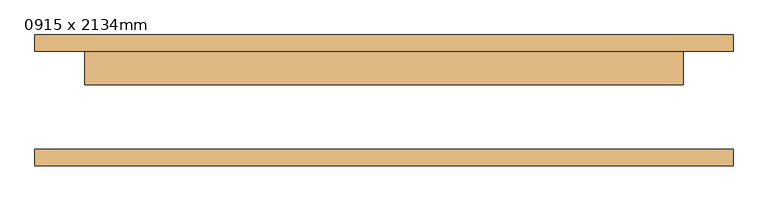
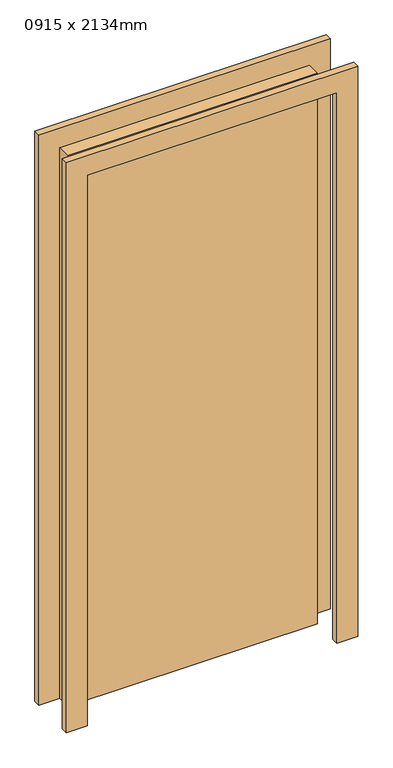
"""IFC4 building model written with IfcOpenShell, lengths in millimetres: door geometry, M_Folha única : 0915 x 2134mm."""

from ifc_helpers import new_model, si_unit, frame, origin, origin_with_axes, place, context, project, spatial, polyline, outline, extrude, source, transform, mapped, element, save


def door_0915_x_2134mm_138fd904(model_context):
    return source(origin(), model_context, "Body", "SweptSolid", [
        extrude(outline(polyline([(2210.0, -533.5), (0.0, -533.5), (0.0, -457.5), (2134.0, -457.5), (2134.0, 457.5), (0.0, 457.5), (0.0, 533.5), (2210.0, 533.5), (2210.0, -533.5)])), frame((0.0, 75.0, 0.0), z_axis=(0.0, 1.0, 0.0), x_axis=(0.0, 0.0, 1.0)), (0.0, 0.0, 1.0), 25.0),
        extrude(outline(polyline([(2210.0, 533.5), (2210.0, -533.5), (0.0, -533.5), (0.0, -457.5), (2134.0, -457.5), (2134.0, 457.5), (0.0, 457.5), (0.0, 533.5), (2210.0, 533.5)])), frame((0.0, -100.0, 0.0), z_axis=(0.0, 1.0, 0.0), x_axis=(0.0, 0.0, 1.0)), (0.0, 0.0, 1.0), 25.0),
        extrude(outline(polyline([(457.5, 24.0), (-457.5, 24.0), (-457.5, 75.0), (457.5, 75.0), (457.5, 24.0)])), origin_with_axes(), (0.0, 0.0, 1.0), 2134.0),
    ])


if __name__ == "__main__":
    model = new_model("IFC4")
    model_context = context("Model", 3, world=origin())
    ifc_project = project(units=[si_unit("LENGTHUNIT", "METRE", prefix="MILLI")], contexts=[model_context])
    site = spatial("IfcSite", under=ifc_project)
    building = spatial("IfcBuilding", under=site)
    placement = place(None, origin())
    door_0915_x_2134mm_shape = door_0915_x_2134mm_138fd904(model_context)
    element("IfcDoor", 1, ObjectType="M_Folha única : 0915 x 2134mm", at=placement, inside=building, context=model_context, shape_type="MappedRepresentation", body=[
        mapped(door_0915_x_2134mm_shape, transform((0.0, 0.0, 0.0), x_axis=(1.0, 0.0, 0.0), y_axis=(0.0, 1.0, 0.0), z_axis=(0.0, 0.0, 1.0))),
    ])
    save(model, "model.ifc")

# Revit data of these elements
# Type "M_Folha única : 0915 x 2134mm"
#   Type Mark = "20"
#   Construction Type Id = "MPORTA"
#   Analytic Construction = "Metal"
#   Thickness = 0.051 m
#   Thermal Resistance (R) = 0.270117 (m²·K)/W
#   Heat Transfer Coefficient (U) = 3.7021 W/(m²·K)
#   Height = 2.134 m
#   Projeção da apara externa = 0.025 m
#   Projeção da apara interna = 0.025 m
#   Largura da apara = 0.076 m
#   Width = 0.915 m
#   Material da porta = Porta - Painel
#   Material da moldura = Porta - Batente
#   Visual Light Transmittance = 0
#   Solar Heat Gain Coefficient = 0
#   Function = (empty or 0)
#   Wall Closure = (empty or 0)
# Element 1 (IfcDoor, "M_Folha única : 0915 x 2134mm")
#   Materials on its faces: "Porta - Batente", "Porta - Painel"
# Materials
#   "Porta - Painel": class "Madeira", colour RGB 210 159 95, transparency 0, Cost = 0
#   "Porta - Batente": class "Diversos", colour RGB 118 70 51, transparency 0, Cost = 0
